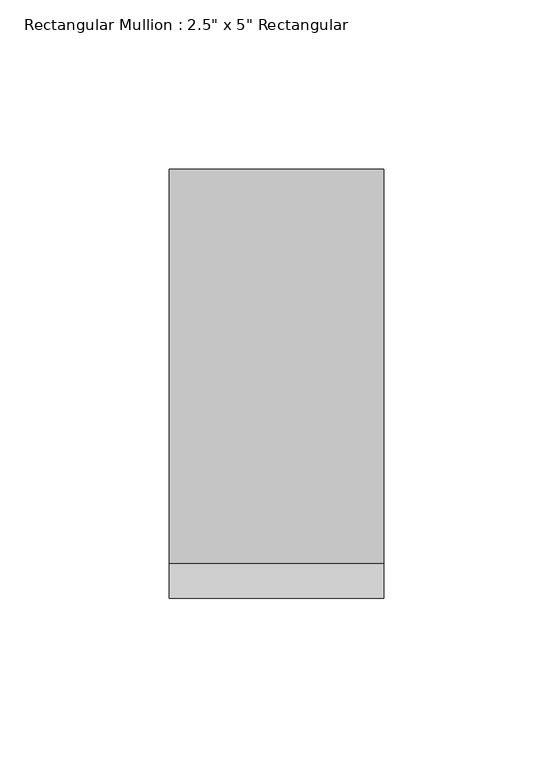
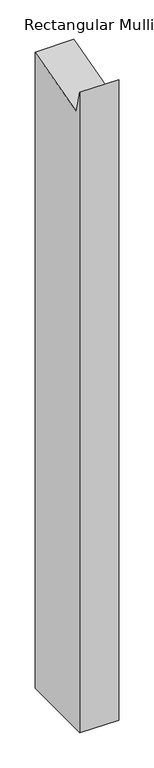
"""IFC4 building model written with IfcOpenShell, lengths in millimetres: member geometry."""

import ifcopenshell
import ifcopenshell.guid

model = None  # the IFC model being written
_history = None  # IfcOwnerHistory: only IFC2X3 demands one
_inside = {}  # id of a spatial element -> (the spatial element, [elements in it])
_under = {}  # id of a project, library or spatial element -> (it, [spatial elements below it])
_declared = {}  # id of a project -> (the project, [libraries it declares])
_typed = {}  # id of a type object -> (the type object, [elements of that type])
_made_of = {}  # id of a material, layer set ... -> (it, [elements and type objects made of it])


def new_model(schema):
    """Start an empty IFC model of exactly this schema.

    Asked for "IFC4X3", IfcOpenShell would pick the latest addendum, in which some entities
    have other attributes; the version numbers below select the first issue.
    IFC2X3 requires an IfcOwnerHistory on every rooted entity: one is made here for all.
    """
    global model, _history
    if schema == "IFC4X3":
        model = ifcopenshell.file(schema_version=(4, 3, 0, 0))
    else:
        model = ifcopenshell.file(schema=schema)
    _inside.clear()
    _under.clear()
    _declared.clear()
    _typed.clear()
    _made_of.clear()
    _history = None
    if model.schema == "IFC2X3":
        org = make("IfcOrganization", Name="unknown")
        user = make(
            "IfcPersonAndOrganization",
            ThePerson=make("IfcPerson", FamilyName="unknown"),
            TheOrganization=org,
        )
        app = make(
            "IfcApplication",
            ApplicationDeveloper=org,
            Version="unknown",
            ApplicationFullName="unknown",
            ApplicationIdentifier="unknown",
        )
        _history = make(
            "IfcOwnerHistory",
            OwningUser=user,
            OwningApplication=app,
            ChangeAction="ADDED",
            CreationDate=0,
        )
    return model


def make(cls, **values):
    """One entity of the class cls with the attributes given. An attribute that is None is left unset."""
    return model.create_entity(
        cls, **{name: value for name, value in values.items() if value is not None}
    )


def rooted(cls, **values):
    """An entity with a GlobalId (a new one), such as an element, a storey or a relation."""
    return make(cls, GlobalId=ifcopenshell.guid.new(), OwnerHistory=_history, **values)


def si_unit(unit_type, name, prefix=None):
    """IfcSIUnit, for example si_unit("LENGTHUNIT", "METRE", prefix="MILLI")."""
    return make("IfcSIUnit", UnitType=unit_type, Prefix=prefix, Name=name)


def assignment(units):
    """IfcUnitAssignment: the units of a project."""
    return None if units is None else make("IfcUnitAssignment", Units=units)


def point(xyz):
    """IfcCartesianPoint."""
    return None if xyz is None else make("IfcCartesianPoint", Coordinates=xyz)


def direction(xyz):
    """IfcDirection."""
    return None if xyz is None else make("IfcDirection", DirectionRatios=xyz)


def frame(location, z_axis=None, x_axis=None):
    """IfcAxis2Placement3D, a coordinate frame: its origin and axes. An axis left out is left unset."""
    return make(
        "IfcAxis2Placement3D",
        Location=point(location),
        Axis=direction(z_axis),
        RefDirection=direction(x_axis),
    )


def origin():
    """The frame at (0, 0, 0) with its axes left unset."""
    return frame((0.0, 0.0, 0.0))


def place(relative_to, where):
    """IfcLocalPlacement: puts the frame where relative to a parent placement (None: the world)."""
    return make(
        "IfcLocalPlacement", PlacementRelTo=relative_to, RelativePlacement=where
    )


def context(
    kind, dimensions, precision=None, world=None, true_north=None, identifier=None
):
    """IfcGeometricRepresentationContext, for example the 3D "Model" context."""
    return make(
        "IfcGeometricRepresentationContext",
        ContextIdentifier=identifier,
        ContextType=kind,
        CoordinateSpaceDimension=dimensions,
        Precision=precision,
        WorldCoordinateSystem=world,
        TrueNorth=true_north,
    )


def project(units=None, contexts=None):
    """IfcProject with its units and contexts."""
    return rooted(
        "IfcProject",
        Name="project",
        RepresentationContexts=contexts,
        UnitsInContext=assignment(units),
    )


def spatial(cls, under=None, at=None, **own):
    """A site, building, storey or space (cls), placed at a placement, below another one or the project."""
    s = rooted(cls, ObjectPlacement=at, **own)
    if under is not None:
        _under.setdefault(under.id(), (under, []))[1].append(s)
    return s


def polyline(points):
    """IfcPolyline through the points."""
    return make("IfcPolyline", Points=[point(p) for p in points])


def outline(outer, holes=None, kind="AREA"):
    """IfcArbitraryClosedProfileDef: a profile drawn as a closed curve; with holes, ...WithVoids."""
    if holes is None:
        return make("IfcArbitraryClosedProfileDef", ProfileType=kind, OuterCurve=outer)
    return make(
        "IfcArbitraryProfileDefWithVoids",
        ProfileType=kind,
        OuterCurve=outer,
        InnerCurves=holes,
    )


def extrude(swept, where, along, depth):
    """IfcExtrudedAreaSolid: the profile swept, set in the frame where, extruded along a direction by depth."""
    return make(
        "IfcExtrudedAreaSolid",
        SweptArea=swept,
        Position=where,
        ExtrudedDirection=direction(along),
        Depth=depth,
    )


def shape(context_of_items, identifier, shape_type, items):
    """IfcShapeRepresentation: the items that make up one representation, for example the "Body"."""
    return make(
        "IfcShapeRepresentation",
        ContextOfItems=context_of_items,
        RepresentationIdentifier=identifier,
        RepresentationType=shape_type,
        Items=items,
    )


def source(mapping_origin, context_of_items, identifier, shape_type, items):
    """IfcRepresentationMap: a shape defined once, which mapped items show again and again."""
    return make(
        "IfcRepresentationMap",
        MappingOrigin=mapping_origin,
        MappedRepresentation=shape(context_of_items, identifier, shape_type, items),
    )


def transform(
    local_origin,
    x_axis=None,
    y_axis=None,
    z_axis=None,
    scale=None,
    scale2=None,
    scale3=None,
    uniform=True,
):
    """IfcCartesianTransformationOperator3D, or its non-uniform kind. x_axis, y_axis, z_axis: its Axis1, 2, 3."""
    if uniform:
        return make(
            "IfcCartesianTransformationOperator3D",
            Axis1=direction(x_axis),
            Axis2=direction(y_axis),
            LocalOrigin=point(local_origin),
            Scale=scale,
            Axis3=direction(z_axis),
        )
    return make(
        "IfcCartesianTransformationOperator3DnonUniform",
        Axis1=direction(x_axis),
        Axis2=direction(y_axis),
        LocalOrigin=point(local_origin),
        Scale=scale,
        Axis3=direction(z_axis),
        Scale2=scale2,
        Scale3=scale3,
    )


def mapped(mapping_source, mapping_target):
    """IfcMappedItem: shows the shape of a source again, moved by a transform."""
    return make(
        "IfcMappedItem", MappingSource=mapping_source, MappingTarget=mapping_target
    )


def made_of(thing, what):
    """Note that an element or type object is made of a material, layer set ...; save() writes the relation."""
    if what is not None:
        _made_of.setdefault(what.id(), (what, []))[1].append(thing)
    return thing


def element(
    cls,
    number,
    at=None,
    inside=None,
    cuts=None,
    type_object=None,
    material=None,
    context=None,
    identifier="Body",
    shape_type=None,
    held_by="IfcProductDefinitionShape",
    body=None,
    shapes=None,
    **own,
):
    """One element of the class cls, such as IfcWall. Its Tag is "e" and its number.

    at: its placement. inside: the storey or other place that contains it. cuts: it is an
    opening in that element (IfcRelVoidsElement). A single representation is given by context,
    identifier, shape_type and body (its items); several are given by shapes. held_by: the class
    of the entity that holds the representations. save() writes the other relations.
    """
    e = rooted(cls, Tag="e%d" % number, ObjectPlacement=at, **own)
    if body is not None:
        shapes = [shape(context, identifier, shape_type, body)]
    if shapes is not None:
        e.Representation = make(held_by, Representations=shapes)
    if inside is not None:
        _inside.setdefault(inside.id(), (inside, []))[1].append(e)
    if cuts is not None:
        rooted(
            "IfcRelVoidsElement", RelatingBuildingElement=cuts, RelatedOpeningElement=e
        )
    if type_object is not None:
        _typed.setdefault(type_object.id(), (type_object, []))[1].append(e)
    return made_of(e, material)


def aggregate(whole, parts):
    """IfcRelAggregates: a whole, such as a stair, and the parts it consists of."""
    return rooted("IfcRelAggregates", RelatingObject=whole, RelatedObjects=parts)


def save(model, path):
    """Write the relations noted so far, then the file.

    IfcRelAggregates (storeys below a building ...), IfcRelContainedInSpatialStructure (elements
    in a storey), IfcRelDefinesByType, IfcRelAssociatesMaterial and IfcRelDeclares: one each for
    every whole, place, type object, material and project.
    """
    for whole, parts in _under.values():
        aggregate(whole, parts)
    for where, things in _inside.values():
        rooted(
            "IfcRelContainedInSpatialStructure",
            RelatedElements=things,
            RelatingStructure=where,
        )
    for kind, things in _typed.values():
        rooted("IfcRelDefinesByType", RelatedObjects=things, RelatingType=kind)
    for what, things in _made_of.values():
        rooted("IfcRelAssociatesMaterial", RelatedObjects=things, RelatingMaterial=what)
    for by, libraries in _declared.values():
        rooted("IfcRelDeclares", RelatingContext=by, RelatedDefinitions=libraries)
    model.write(path)


def member_30683c4a(model_context):
    return source(origin(), model_context, "Body", "SweptSolid", [
        extrude(outline(polyline([(-63.5, 23.3900664), (-53.1187853, -15.3531543), (63.5, 15.894755), (63.5, -1088.0706742), (-63.5, -1088.0706742), (-63.5, 23.3900664)])), frame((-63.5, 0.0, 0.0), z_axis=(1.0, 0.0, 0.0), x_axis=(0.0, 1.0, 0.0)), (0.0, 0.0, 1.0), 63.5),
    ])


if __name__ == "__main__":
    model = new_model("IFC4")
    model_context = context("Model", 3, world=origin())
    ifc_project = project(units=[si_unit("LENGTHUNIT", "METRE", prefix="MILLI")], contexts=[model_context])
    site = spatial("IfcSite", under=ifc_project)
    building = spatial("IfcBuilding", under=site)
    placement = place(None, origin())
    member_shape = member_30683c4a(model_context)
    element("IfcMember", 1, ObjectType="Rectangular Mullion : 2.5\" x 5\" Rectangular", at=placement, inside=building, context=model_context, shape_type="MappedRepresentation", body=[
        mapped(member_shape, transform((0.0, 0.0, 0.0), x_axis=(1.0, 0.0, 0.0), y_axis=(0.0, 1.0, 0.0), z_axis=(0.0, 0.0, 1.0))),
    ])
    save(model, "model.ifc")

# Revit data of these elements
# Type "Rectangular Mullion : 2.5\" x 5\" Rectangular"
#   built-in parameter 1007304 = 0.416667 (stored number, unit not read)
#   built-in parameter 1007301 = 0.104167 (stored number, unit not read)
#   built-in parameter 1007300 = 0.104167 (stored number, unit not read)
# Element 1 (IfcMember, "Rectangular Mullion : 2.5\" x 5\" Rectangular")
#   Materials on its faces: "Aluminum"
# Materials
#   "Aluminum": class "Metal", colour RGB 247 247 247, transparency 0, Description = "Aluminum 6061", Cost = 0
